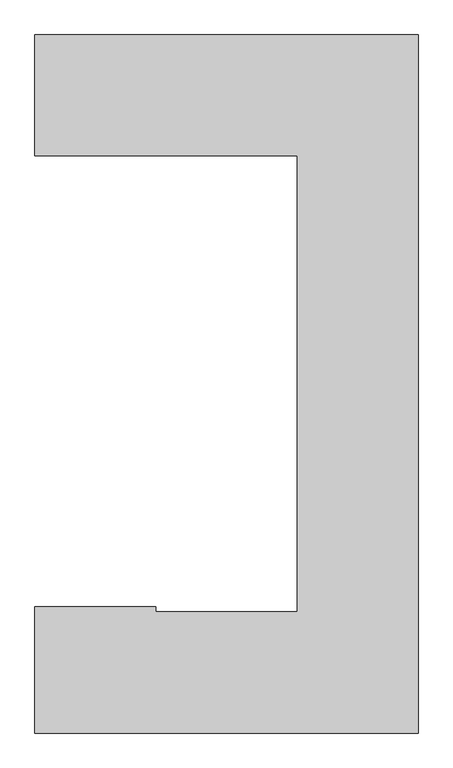
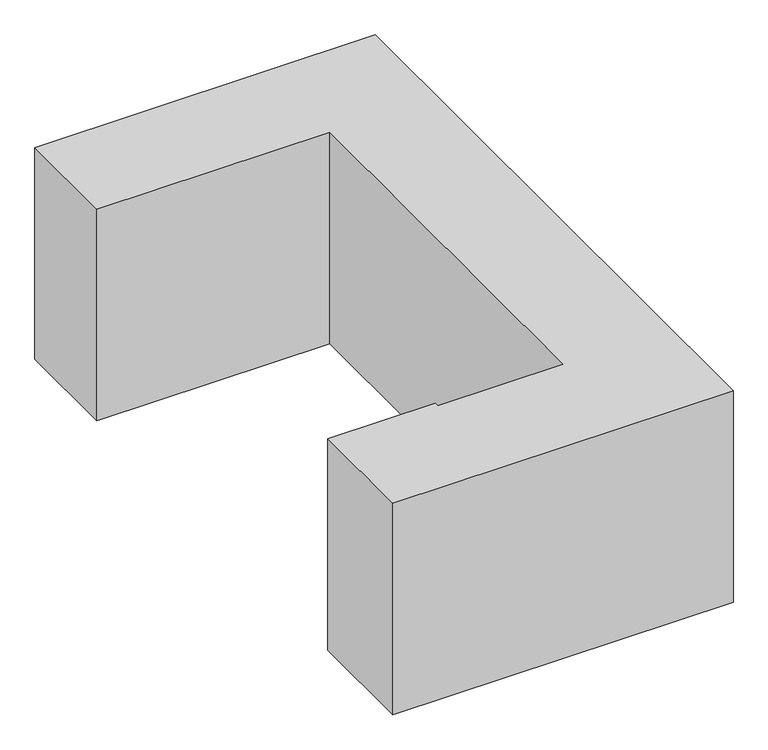
"""IFC4 building model written with IfcOpenShell, lengths in millimetres: proxy geometry, 0_3d_modell."""

from ifc_helpers import new_model, si_unit, origin, origin_with_axes, place, context, project, spatial, polyline, outline, extrude, source, transform, mapped, element, save


def generic_models_6dfd55e4(model_context):
    return source(origin(), model_context, "Body", "SweptSolid", [
        extrude(outline(polyline([(3800.0, 6925.0), (3800.0, 0.0), (0.0, 0.0), (0.0, 1255.0837476), (1198.7770373, 1255.0033532), (1198.7770373, 1205.0), (2600.0, 1205.0), (2600.0, 5725.0), (0.0, 5725.0), (0.0, 6925.0), (3800.0, 6925.0)])), origin_with_axes(), (0.0, 0.0, 1.0), 2500.0),
    ])


if __name__ == "__main__":
    model = new_model("IFC4")
    model_context = context("Model", 3, world=origin())
    ifc_project = project(units=[si_unit("LENGTHUNIT", "METRE", prefix="MILLI")], contexts=[model_context])
    site = spatial("IfcSite", under=ifc_project)
    building = spatial("IfcBuilding", under=site)
    placement = place(None, origin())
    generic_models_shape = generic_models_6dfd55e4(model_context)
    element("IfcBuildingElementProxy", 1, Name="0_3d_modell", ObjectType="0_3d_modell", at=placement, inside=building, context=model_context, shape_type="MappedRepresentation", body=[
        mapped(generic_models_shape, transform((0.0, 0.0, 0.0), x_axis=(1.0, 0.0, 0.0), y_axis=(0.0, 1.0, 0.0), z_axis=(0.0, 0.0, 1.0))),
    ])
    save(model, "model.ifc")

# Revit data of these elements
# Element 1 (IfcBuildingElementProxy, "0_3d_modell")
#   Materials on its faces: "*1"
# Materials
#   "*1": class "Unassigned", colour RGB 175 175 175, transparency 0
